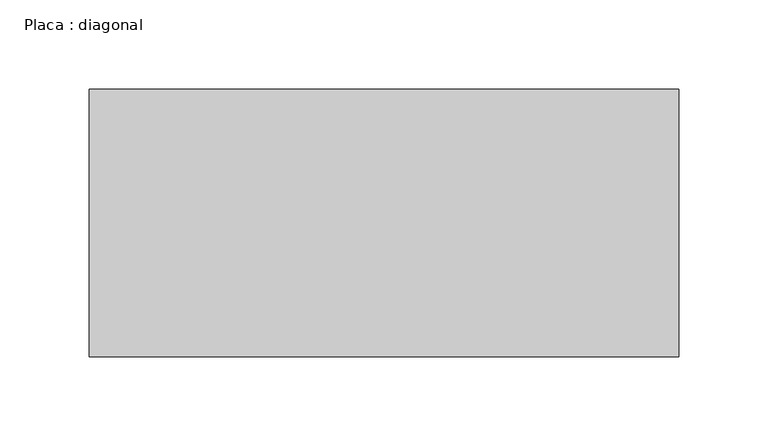
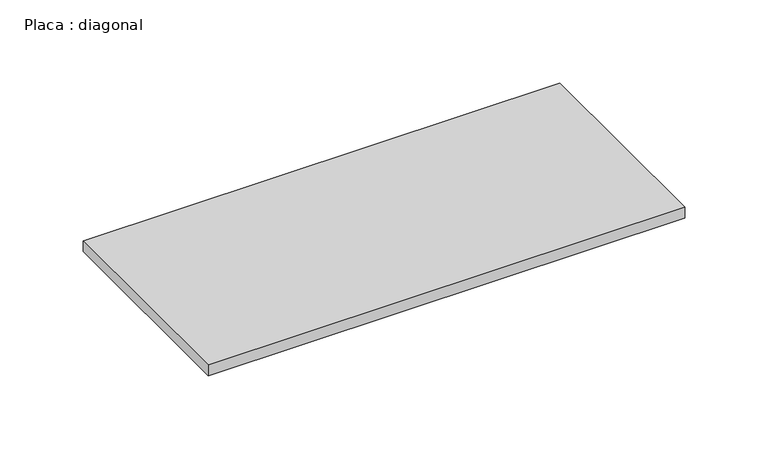
"""IFC4 building model written with IfcOpenShell, lengths in millimetres: beam geometry, Placa : diagonal."""

from ifc_helpers import new_model, si_unit, frame, origin, place, context, project, spatial, polyline, outline, extrude, source, transform, mapped, element, save


def placa_diagonal_dc3ee5ab(model_context):
    return source(origin(), model_context, "Body", "SweptSolid", [
        extrude(outline(polyline([(165.4962727, 75.0), (165.4962727, -75.0), (-165.1705214, -75.0), (-165.1705214, 75.0), (165.4962727, 75.0)])), frame((0.0, 0.0, -4.0), z_axis=(0.0, 0.0, 1.0), x_axis=(1.0, 0.0, 0.0)), (0.0, 0.0, 1.0), 8.0),
    ])


if __name__ == "__main__":
    model = new_model("IFC4")
    model_context = context("Model", 3, world=origin())
    ifc_project = project(units=[si_unit("LENGTHUNIT", "METRE", prefix="MILLI")], contexts=[model_context])
    site = spatial("IfcSite", under=ifc_project)
    building = spatial("IfcBuilding", under=site)
    placement = place(None, origin())
    placa_diagonal_shape = placa_diagonal_dc3ee5ab(model_context)
    element("IfcBeam", 1, ObjectType="Placa : diagonal", at=placement, inside=building, context=model_context, shape_type="MappedRepresentation", body=[
        mapped(placa_diagonal_shape, transform((0.0, 0.0, 0.0), x_axis=(1.0, 0.0, 0.0), y_axis=(0.0, 1.0, 0.0), z_axis=(0.0, 0.0, 1.0))),
    ])
    save(model, "model.ifc")

# Revit data of these elements
# Type "Placa : diagonal"
#   W = 0
#   Length [instance default] = 1.50 m
#   b = 0.15 m
#   d = 0.008 m
#   A = 0 m²
#   Structural Material [instance default] = Aço, 45-345
# Element 1 (IfcBeam, "Placa : diagonal")
#   Materials on its faces: "Aço, 45-345"
# Materials
#   "Aço, 45-345": class "Metal", colour RGB 247 247 247, transparency 0, Description = "Aço 345 MPa", Cost = 0
